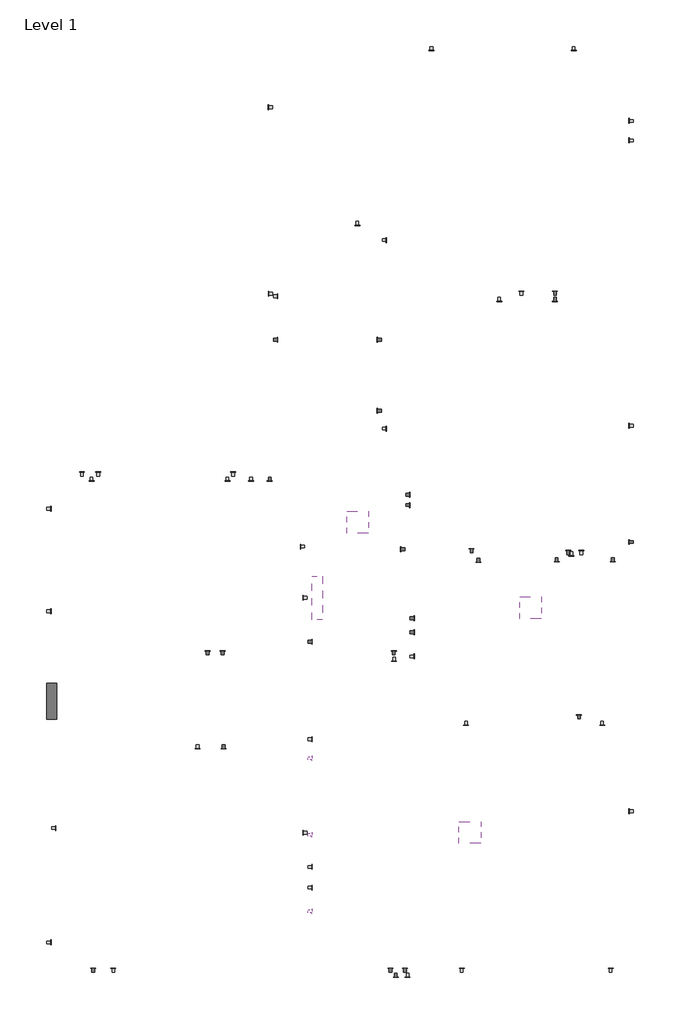
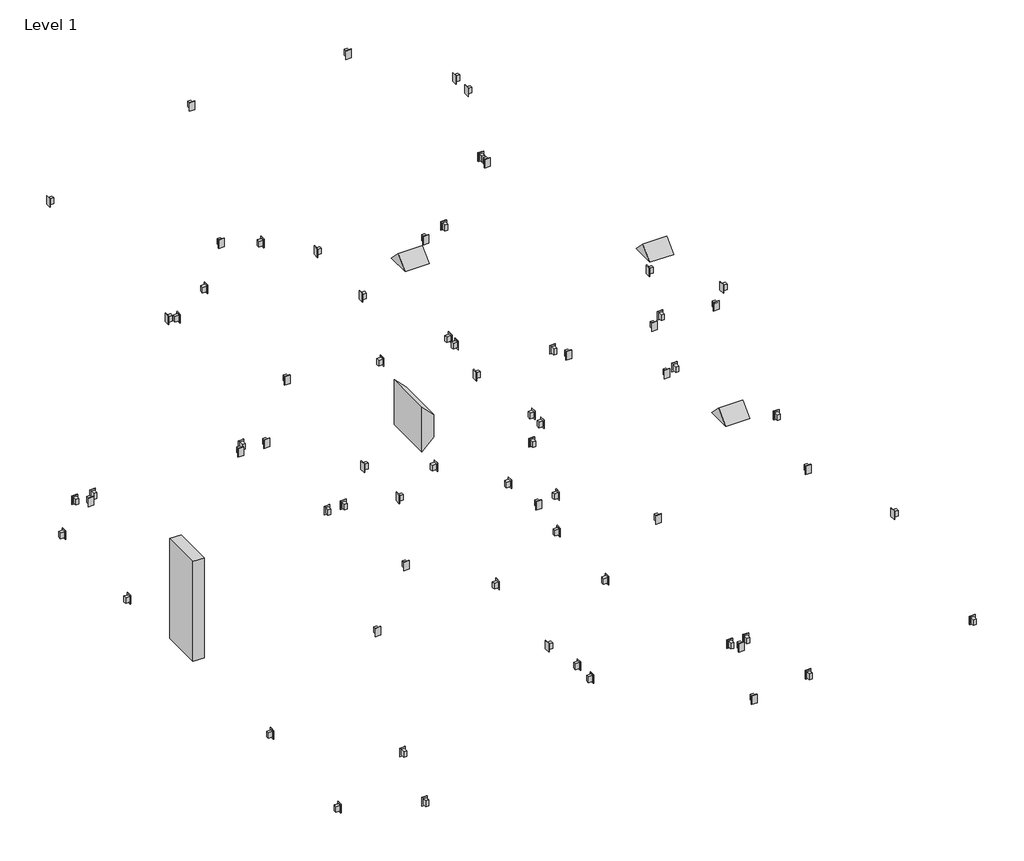
# One storey: 48 proxies, 16 switching devices, 8 electric appliances, 4 light fixtures.
"""IFC4 building model written with IfcOpenShell, lengths in millimetres."""

import ifcopenshell
import ifcopenshell.guid

model = None  # the IFC model being written
_history = None  # IfcOwnerHistory: only IFC2X3 demands one
_inside = {}  # id of a spatial element -> (the spatial element, [elements in it])
_under = {}  # id of a project, library or spatial element -> (it, [spatial elements below it])
_declared = {}  # id of a project -> (the project, [libraries it declares])
_typed = {}  # id of a type object -> (the type object, [elements of that type])
_made_of = {}  # id of a material, layer set ... -> (it, [elements and type objects made of it])


def new_model(schema):
    """Start an empty IFC model of exactly this schema.

    Asked for "IFC4X3", IfcOpenShell would pick the latest addendum, in which some entities
    have other attributes; the version numbers below select the first issue.
    IFC2X3 requires an IfcOwnerHistory on every rooted entity: one is made here for all.
    """
    global model, _history
    if schema == "IFC4X3":
        model = ifcopenshell.file(schema_version=(4, 3, 0, 0))
    else:
        model = ifcopenshell.file(schema=schema)
    _inside.clear()
    _under.clear()
    _declared.clear()
    _typed.clear()
    _made_of.clear()
    _history = None
    if model.schema == "IFC2X3":
        org = make("IfcOrganization", Name="unknown")
        user = make(
            "IfcPersonAndOrganization",
            ThePerson=make("IfcPerson", FamilyName="unknown"),
            TheOrganization=org,
        )
        app = make(
            "IfcApplication",
            ApplicationDeveloper=org,
            Version="unknown",
            ApplicationFullName="unknown",
            ApplicationIdentifier="unknown",
        )
        _history = make(
            "IfcOwnerHistory",
            OwningUser=user,
            OwningApplication=app,
            ChangeAction="ADDED",
            CreationDate=0,
        )
    return model


def make(cls, **values):
    """One entity of the class cls with the attributes given. An attribute that is None is left unset."""
    return model.create_entity(
        cls, **{name: value for name, value in values.items() if value is not None}
    )


def rooted(cls, **values):
    """An entity with a GlobalId (a new one), such as an element, a storey or a relation."""
    return make(cls, GlobalId=ifcopenshell.guid.new(), OwnerHistory=_history, **values)


def si_unit(unit_type, name, prefix=None):
    """IfcSIUnit, for example si_unit("LENGTHUNIT", "METRE", prefix="MILLI")."""
    return make("IfcSIUnit", UnitType=unit_type, Prefix=prefix, Name=name)


def assignment(units):
    """IfcUnitAssignment: the units of a project."""
    return None if units is None else make("IfcUnitAssignment", Units=units)


def point(xyz):
    """IfcCartesianPoint."""
    return None if xyz is None else make("IfcCartesianPoint", Coordinates=xyz)


def direction(xyz):
    """IfcDirection."""
    return None if xyz is None else make("IfcDirection", DirectionRatios=xyz)


def frame(location, z_axis=None, x_axis=None):
    """IfcAxis2Placement3D, a coordinate frame: its origin and axes. An axis left out is left unset."""
    return make(
        "IfcAxis2Placement3D",
        Location=point(location),
        Axis=direction(z_axis),
        RefDirection=direction(x_axis),
    )


def origin():
    """The frame at (0, 0, 0) with its axes left unset."""
    return frame((0.0, 0.0, 0.0))


def origin_with_axes():
    """The frame at (0, 0, 0) with the z axis (0, 0, 1) and the x axis (1, 0, 0) written out."""
    return frame((0.0, 0.0, 0.0), z_axis=(0.0, 0.0, 1.0), x_axis=(1.0, 0.0, 0.0))


def place(relative_to, where):
    """IfcLocalPlacement: puts the frame where relative to a parent placement (None: the world)."""
    return make(
        "IfcLocalPlacement", PlacementRelTo=relative_to, RelativePlacement=where
    )


def context(
    kind, dimensions, precision=None, world=None, true_north=None, identifier=None
):
    """IfcGeometricRepresentationContext, for example the 3D "Model" context."""
    return make(
        "IfcGeometricRepresentationContext",
        ContextIdentifier=identifier,
        ContextType=kind,
        CoordinateSpaceDimension=dimensions,
        Precision=precision,
        WorldCoordinateSystem=world,
        TrueNorth=true_north,
    )


def project(units=None, contexts=None):
    """IfcProject with its units and contexts."""
    return rooted(
        "IfcProject",
        Name="project",
        RepresentationContexts=contexts,
        UnitsInContext=assignment(units),
    )


def spatial(cls, under=None, at=None, **own):
    """A site, building, storey or space (cls), placed at a placement, below another one or the project."""
    s = rooted(cls, ObjectPlacement=at, **own)
    if under is not None:
        _under.setdefault(under.id(), (under, []))[1].append(s)
    return s


def polyline(points):
    """IfcPolyline through the points."""
    return make("IfcPolyline", Points=[point(p) for p in points])


def outline(outer, holes=None, kind="AREA"):
    """IfcArbitraryClosedProfileDef: a profile drawn as a closed curve; with holes, ...WithVoids."""
    if holes is None:
        return make("IfcArbitraryClosedProfileDef", ProfileType=kind, OuterCurve=outer)
    return make(
        "IfcArbitraryProfileDefWithVoids",
        ProfileType=kind,
        OuterCurve=outer,
        InnerCurves=holes,
    )


def extrude(swept, where, along, depth):
    """IfcExtrudedAreaSolid: the profile swept, set in the frame where, extruded along a direction by depth."""
    return make(
        "IfcExtrudedAreaSolid",
        SweptArea=swept,
        Position=where,
        ExtrudedDirection=direction(along),
        Depth=depth,
    )


def shape(context_of_items, identifier, shape_type, items):
    """IfcShapeRepresentation: the items that make up one representation, for example the "Body"."""
    return make(
        "IfcShapeRepresentation",
        ContextOfItems=context_of_items,
        RepresentationIdentifier=identifier,
        RepresentationType=shape_type,
        Items=items,
    )


def source(mapping_origin, context_of_items, identifier, shape_type, items):
    """IfcRepresentationMap: a shape defined once, which mapped items show again and again."""
    return make(
        "IfcRepresentationMap",
        MappingOrigin=mapping_origin,
        MappedRepresentation=shape(context_of_items, identifier, shape_type, items),
    )


def transform(
    local_origin,
    x_axis=None,
    y_axis=None,
    z_axis=None,
    scale=None,
    scale2=None,
    scale3=None,
    uniform=True,
):
    """IfcCartesianTransformationOperator3D, or its non-uniform kind. x_axis, y_axis, z_axis: its Axis1, 2, 3."""
    if uniform:
        return make(
            "IfcCartesianTransformationOperator3D",
            Axis1=direction(x_axis),
            Axis2=direction(y_axis),
            LocalOrigin=point(local_origin),
            Scale=scale,
            Axis3=direction(z_axis),
        )
    return make(
        "IfcCartesianTransformationOperator3DnonUniform",
        Axis1=direction(x_axis),
        Axis2=direction(y_axis),
        LocalOrigin=point(local_origin),
        Scale=scale,
        Axis3=direction(z_axis),
        Scale2=scale2,
        Scale3=scale3,
    )


def mapped(mapping_source, mapping_target):
    """IfcMappedItem: shows the shape of a source again, moved by a transform."""
    return make(
        "IfcMappedItem", MappingSource=mapping_source, MappingTarget=mapping_target
    )


def made_of(thing, what):
    """Note that an element or type object is made of a material, layer set ...; save() writes the relation."""
    if what is not None:
        _made_of.setdefault(what.id(), (what, []))[1].append(thing)
    return thing


def element(
    cls,
    number,
    at=None,
    inside=None,
    cuts=None,
    type_object=None,
    material=None,
    context=None,
    identifier="Body",
    shape_type=None,
    held_by="IfcProductDefinitionShape",
    body=None,
    shapes=None,
    **own,
):
    """One element of the class cls, such as IfcWall. Its Tag is "e" and its number.

    at: its placement. inside: the storey or other place that contains it. cuts: it is an
    opening in that element (IfcRelVoidsElement). A single representation is given by context,
    identifier, shape_type and body (its items); several are given by shapes. held_by: the class
    of the entity that holds the representations. save() writes the other relations.
    """
    e = rooted(cls, Tag="e%d" % number, ObjectPlacement=at, **own)
    if body is not None:
        shapes = [shape(context, identifier, shape_type, body)]
    if shapes is not None:
        e.Representation = make(held_by, Representations=shapes)
    if inside is not None:
        _inside.setdefault(inside.id(), (inside, []))[1].append(e)
    if cuts is not None:
        rooted(
            "IfcRelVoidsElement", RelatingBuildingElement=cuts, RelatedOpeningElement=e
        )
    if type_object is not None:
        _typed.setdefault(type_object.id(), (type_object, []))[1].append(e)
    return made_of(e, material)


def aggregate(whole, parts):
    """IfcRelAggregates: a whole, such as a stair, and the parts it consists of."""
    return rooted("IfcRelAggregates", RelatingObject=whole, RelatedObjects=parts)


def save(model, path):
    """Write the relations noted so far, then the file.

    IfcRelAggregates (storeys below a building ...), IfcRelContainedInSpatialStructure (elements
    in a storey), IfcRelDefinesByType, IfcRelAssociatesMaterial and IfcRelDeclares: one each for
    every whole, place, type object, material and project.
    """
    for whole, parts in _under.values():
        aggregate(whole, parts)
    for where, things in _inside.values():
        rooted(
            "IfcRelContainedInSpatialStructure",
            RelatedElements=things,
            RelatingStructure=where,
        )
    for kind, things in _typed.values():
        rooted("IfcRelDefinesByType", RelatedObjects=things, RelatingType=kind)
    for what, things in _made_of.values():
        rooted("IfcRelAssociatesMaterial", RelatedObjects=things, RelatingMaterial=what)
    for by, libraries in _declared.values():
        rooted("IfcRelDeclares", RelatingContext=by, RelatedDefinitions=libraries)
    model.write(path)


def duplex_receptacle_gfci_10251bba(model_context):
    return source(origin(), model_context, "Body", "SweptSolid", [
        extrude(outline(polyline([(19.05, 38.1), (19.05, -38.1), (-19.05, -38.1), (-19.05, 38.1), (19.05, 38.1)])), frame((0.0, 0.0, -53.975), z_axis=(0.0, 0.0, 1.0), x_axis=(1.0, 0.0, 0.0)), (0.0, 0.0, 1.0), 53.975),
        extrude(outline(polyline([(34.925, 57.15), (34.925, -57.15), (-34.925, -57.15), (-34.925, 57.15), (34.925, 57.15)])), origin_with_axes(), (0.0, 0.0, 1.0), 4.7625),
    ])


def lighting_and_appliance_panelboard_208v_mlo_400_a_bd3ac378(model_context):
    return source(origin(), model_context, "Body", "SweptSolid", [
        extrude(outline(polyline([(254.0, 673.1), (254.0, -673.1), (-254.0, -673.1), (-254.0, 673.1), (254.0, 673.1)])), frame((0.0, 0.0, -146.05), z_axis=(0.0, 0.0, 1.0), x_axis=(1.0, 0.0, 0.0)), (0.0, 0.0, 1.0), 146.05),
    ])


def data_outlet_plain_367a9a66(model_context):
    return source(origin(), model_context, "Body", "SweptSolid", [
        extrude(outline(polyline([(34.925, 57.15), (34.925, -57.15), (-34.925, -57.15), (-34.925, 57.15), (34.925, 57.15)])), origin_with_axes(), (0.0, 0.0, 1.0), 4.7625),
        extrude(outline(polyline([(19.05, 38.1), (19.05, -38.1), (-19.05, -38.1), (-19.05, 38.1), (19.05, 38.1)])), frame((0.0, 0.0, -53.975), z_axis=(0.0, 0.0, 1.0), x_axis=(1.0, 0.0, 0.0)), (0.0, 0.0, 1.0), 53.975),
    ])


def plain_recessed_lighting_fixture_2x2_120_2107ce2d(model_context):
    return source(origin(), model_context, "Body", "SweptSolid", [
        extrude(outline(polyline([(-609.6, 0.0), (0.0, 0.0), (-152.4, -152.4), (-457.2, -152.4), (-609.6, 0.0)])), frame((0.0, 0.0, 0.0), z_axis=(1.0, 0.0, 0.0), x_axis=(0.0, 1.0, 0.0)), (0.0, 0.0, 1.0), 609.6),
    ])


def plain_recessed_lighting_fixture_large_bulb_b9741ada(model_context):
    return source(origin(), model_context, "Body", "SweptSolid", [
        extrude(outline(polyline([(-304.8, 0.0), (0.0, 0.0), (-152.4, -152.4), (-304.8, 0.0)])), frame((0.0, 0.0, 0.0), z_axis=(1.0, 0.0, 0.0), x_axis=(0.0, 1.0, 0.0)), (0.0, 0.0, 1.0), 304.8),
    ])


model = new_model("IFC4")

# Units and contexts
model_context = context("Model", 3, world=origin())
ifc_project = project(units=[si_unit("LENGTHUNIT", "METRE", prefix="MILLI")], contexts=[model_context])

# Site, building, storey
site = spatial("IfcSite", under=ifc_project)
building = spatial("IfcBuilding", under=site)
storey = spatial("IfcBuildingStorey", under=building, Name="Level 1", Elevation=0.0)

# Proxies
placement = place(None, origin())
duplex_receptacle_gfci_shape = duplex_receptacle_gfci_10251bba(model_context)
element("IfcBuildingElementProxy", 1, Name="Duplex Receptacle : GFCI", ObjectType="Duplex Receptacle : GFCI", at=placement, inside=storey, context=model_context, shape_type="MappedRepresentation", body=[
    mapped(duplex_receptacle_gfci_shape, transform((-384.264748, 4509.2322925, 1219.2), x_axis=(0.0, 1.0, 0.0), y_axis=(0.0, 0.0, 1.0), z_axis=(1.0, 0.0, 0.0))),
])
element("IfcBuildingElementProxy", 2, Name="Duplex Receptacle : GFCI", ObjectType="Duplex Receptacle : GFCI", at=placement, inside=storey, context=model_context, shape_type="MappedRepresentation", body=[
    mapped(duplex_receptacle_gfci_shape, transform((-384.264748, 4707.743975, 1219.2), x_axis=(0.0, 1.0, 0.0), y_axis=(0.0, 0.0, 1.0), z_axis=(1.0, 0.0, 0.0))),
])
element("IfcBuildingElementProxy", 3, Name="Duplex Receptacle : GFCI", ObjectType="Duplex Receptacle : GFCI", at=placement, inside=storey, context=model_context, shape_type="MappedRepresentation", body=[
    mapped(duplex_receptacle_gfci_shape, transform((520.3675151, 5493.8871474, 1219.2), x_axis=(1.0, 0.0, 0.0), y_axis=(0.0, 0.0, 1.0), z_axis=(0.0, -1.0, 0.0))),
])
element("IfcBuildingElementProxy", 4, Name="Duplex Receptacle : GFCI", ObjectType="Duplex Receptacle : GFCI", at=placement, inside=storey, context=model_context, shape_type="MappedRepresentation", body=[
    mapped(duplex_receptacle_gfci_shape, transform((1616.819892, 5500.2371474, 1219.2), x_axis=(1.0, 0.0, 0.0), y_axis=(0.0, 0.0, 1.0), z_axis=(0.0, -1.0, 0.0))),
])
element("IfcBuildingElementProxy", 5, Name="Duplex Receptacle : GFCI", ObjectType="Duplex Receptacle : GFCI", at=placement, inside=storey, context=model_context, shape_type="MappedRepresentation", body=[
    mapped(duplex_receptacle_gfci_shape, transform((2401.5903749, 5500.2371474, 1219.2), x_axis=(1.0, 0.0, 0.0), y_axis=(0.0, 0.0, 1.0), z_axis=(0.0, -1.0, 0.0))),
])
element("IfcBuildingElementProxy", 6, Name="Duplex Receptacle : GFCI", ObjectType="Duplex Receptacle : GFCI", at=placement, inside=storey, context=model_context, shape_type="MappedRepresentation", body=[
    mapped(duplex_receptacle_gfci_shape, transform((-444.589748, 6434.9811372, 1219.2), x_axis=(0.0, 1.0, 0.0), y_axis=(0.0, 0.0, 1.0), z_axis=(1.0, 0.0, 0.0))),
])
element("IfcBuildingElementProxy", 7, Name="Duplex Receptacle : GFCI", ObjectType="Duplex Receptacle : GFCI", at=placement, inside=storey, context=model_context, shape_type="MappedRepresentation", body=[
    mapped(duplex_receptacle_gfci_shape, transform((-444.589748, 6292.1269358, 1219.2), x_axis=(0.0, 1.0, 0.0), y_axis=(0.0, 0.0, 1.0), z_axis=(1.0, 0.0, 0.0))),
])
element("IfcBuildingElementProxy", 8, Name="Duplex Receptacle : GFCI", ObjectType="Duplex Receptacle : GFCI", at=placement, inside=storey, context=model_context, shape_type="MappedRepresentation", body=[
    mapped(duplex_receptacle_gfci_shape, transform((423.8945479, 5678.0371474, 1219.2), x_axis=(-1.0, 0.0, 0.0), y_axis=(0.0, 0.0, 1.0), z_axis=(0.0, 1.0, 0.0))),
])
element("IfcBuildingElementProxy", 9, Name="Duplex Receptacle : GFCI", ObjectType="Duplex Receptacle : GFCI", at=placement, inside=storey, context=model_context, shape_type="MappedRepresentation", body=[
    mapped(duplex_receptacle_gfci_shape, transform((1778.2265871, 5652.6371474, 1219.2), x_axis=(-1.0, 0.0, 0.0), y_axis=(0.0, 0.0, 1.0), z_axis=(0.0, 1.0, 0.0))),
])
element("IfcBuildingElementProxy", 10, Name="Duplex Receptacle : GFCI", ObjectType="Duplex Receptacle : GFCI", at=placement, inside=storey, context=model_context, shape_type="MappedRepresentation", body=[
    mapped(duplex_receptacle_gfci_shape, transform((2635.160252, 5774.512362, 1219.2), x_axis=(0.0, -1.0, 0.0), y_axis=(0.0, 0.0, 1.0), z_axis=(-1.0, 0.0, 0.0))),
])
element("IfcBuildingElementProxy", 11, Name="Duplex Receptacle : GFCI", ObjectType="Duplex Receptacle : GFCI", at=placement, inside=storey, context=model_context, shape_type="MappedRepresentation", body=[
    mapped(duplex_receptacle_gfci_shape, transform((-1816.189748, 4378.2462129, 1219.2), x_axis=(0.0, 1.0, 0.0), y_axis=(0.0, 0.0, 1.0), z_axis=(1.0, 0.0, 0.0))),
])
element("IfcBuildingElementProxy", 12, Name="Duplex Receptacle : Standard", ObjectType="Duplex Receptacle : Standard", at=placement, inside=storey, context=model_context, shape_type="MappedRepresentation", body=[
    mapped(duplex_receptacle_gfci_shape, transform((-5473.789748, 4805.3855798, 457.2), x_axis=(0.0, 1.0, 0.0), y_axis=(0.0, 0.0, 1.0), z_axis=(1.0, 0.0, 0.0))),
])
element("IfcBuildingElementProxy", 13, Name="Duplex Receptacle : Standard", ObjectType="Duplex Receptacle : Standard", at=placement, inside=storey, context=model_context, shape_type="MappedRepresentation", body=[
    mapped(duplex_receptacle_gfci_shape, transform((-5473.789748, 6239.7970199, 457.2), x_axis=(0.0, 1.0, 0.0), y_axis=(0.0, 0.0, 1.0), z_axis=(1.0, 0.0, 0.0))),
])
element("IfcBuildingElementProxy", 14, Name="Duplex Receptacle : Standard", ObjectType="Duplex Receptacle : Standard", at=placement, inside=storey, context=model_context, shape_type="MappedRepresentation", body=[
    mapped(duplex_receptacle_gfci_shape, transform((-4904.2560493, 6630.4078904, 457.2), x_axis=(1.0, 0.0, 0.0), y_axis=(0.0, 0.0, 1.0), z_axis=(0.0, -1.0, 0.0))),
])
element("IfcBuildingElementProxy", 15, Name="Duplex Receptacle : Standard", ObjectType="Duplex Receptacle : Standard", at=placement, inside=storey, context=model_context, shape_type="MappedRepresentation", body=[
    mapped(duplex_receptacle_gfci_shape, transform((-2998.0299372, 6630.4078904, 457.2), x_axis=(1.0, 0.0, 0.0), y_axis=(0.0, 0.0, 1.0), z_axis=(0.0, -1.0, 0.0))),
])
element("IfcBuildingElementProxy", 16, Name="Duplex Receptacle : Standard", ObjectType="Duplex Receptacle : Standard", at=placement, inside=storey, context=model_context, shape_type="MappedRepresentation", body=[
    mapped(duplex_receptacle_gfci_shape, transform((-2666.1000171, 6630.4078904, 457.2), x_axis=(1.0, 0.0, 0.0), y_axis=(0.0, 0.0, 1.0), z_axis=(0.0, -1.0, 0.0))),
])
element("IfcBuildingElementProxy", 17, Name="Duplex Receptacle : Standard", ObjectType="Duplex Receptacle : Standard", at=placement, inside=storey, context=model_context, shape_type="MappedRepresentation", body=[
    mapped(duplex_receptacle_gfci_shape, transform((-1936.839748, 4995.0598198, 457.2), x_axis=(0.0, -1.0, 0.0), y_axis=(0.0, 0.0, 1.0), z_axis=(-1.0, 0.0, 0.0))),
])
element("IfcBuildingElementProxy", 18, Name="Duplex Receptacle : Standard", ObjectType="Duplex Receptacle : Standard", at=placement, inside=storey, context=model_context, shape_type="MappedRepresentation", body=[
    mapped(duplex_receptacle_gfci_shape, transform((-3414.9283858, 2880.8621474, 457.2), x_axis=(1.0, 0.0, 0.0), y_axis=(0.0, 0.0, 1.0), z_axis=(0.0, -1.0, 0.0))),
])
element("IfcBuildingElementProxy", 19, Name="Duplex Receptacle : Standard", ObjectType="Duplex Receptacle : Standard", at=placement, inside=storey, context=model_context, shape_type="MappedRepresentation", body=[
    mapped(duplex_receptacle_gfci_shape, transform((-1936.839748, 1703.0761834, 457.2), x_axis=(0.0, -1.0, 0.0), y_axis=(0.0, 0.0, 1.0), z_axis=(-1.0, 0.0, 0.0))),
])
element("IfcBuildingElementProxy", 20, Name="Duplex Receptacle : Standard", ObjectType="Duplex Receptacle : Standard", at=placement, inside=storey, context=model_context, shape_type="MappedRepresentation", body=[
    mapped(duplex_receptacle_gfci_shape, transform((-4597.0361882, -198.8878526, 457.2), x_axis=(-1.0, 0.0, 0.0), y_axis=(0.0, 0.0, 1.0), z_axis=(0.0, 1.0, 0.0))),
])
element("IfcBuildingElementProxy", 21, Name="Duplex Receptacle : Standard", ObjectType="Duplex Receptacle : Standard", at=placement, inside=storey, context=model_context, shape_type="MappedRepresentation", body=[
    mapped(duplex_receptacle_gfci_shape, transform((-5407.114748, 1768.3250081, 457.2), x_axis=(0.0, 1.0, 0.0), y_axis=(0.0, 0.0, 1.0), z_axis=(1.0, 0.0, 0.0))),
])
element("IfcBuildingElementProxy", 22, Name="Duplex Receptacle : Standard", ObjectType="Duplex Receptacle : Standard", at=placement, inside=storey, context=model_context, shape_type="MappedRepresentation", body=[
    mapped(duplex_receptacle_gfci_shape, transform((-1816.189748, 2744.9323475, 1981.2), x_axis=(0.0, 1.0, 0.0), y_axis=(0.0, 0.0, 1.0), z_axis=(1.0, 0.0, 0.0))),
])
element("IfcBuildingElementProxy", 23, Name="Duplex Receptacle : Standard", ObjectType="Duplex Receptacle : Standard", at=placement, inside=storey, context=model_context, shape_type="MappedRepresentation", body=[
    mapped(duplex_receptacle_gfci_shape, transform((-1816.189748, 1673.8457407, 1981.2), x_axis=(0.0, 1.0, 0.0), y_axis=(0.0, 0.0, 1.0), z_axis=(1.0, 0.0, 0.0))),
])
element("IfcBuildingElementProxy", 24, Name="Duplex Receptacle : Standard", ObjectType="Duplex Receptacle : Standard", at=placement, inside=storey, context=model_context, shape_type="MappedRepresentation", body=[
    mapped(duplex_receptacle_gfci_shape, transform((-1816.189748, 602.759134, 1981.2), x_axis=(0.0, 1.0, 0.0), y_axis=(0.0, 0.0, 1.0), z_axis=(1.0, 0.0, 0.0))),
])
element("IfcBuildingElementProxy", 25, Name="Duplex Receptacle : Standard", ObjectType="Duplex Receptacle : Standard", at=placement, inside=storey, context=model_context, shape_type="MappedRepresentation", body=[
    mapped(duplex_receptacle_gfci_shape, transform((-1816.189748, 1223.3093109, 457.2), x_axis=(0.0, 1.0, 0.0), y_axis=(0.0, 0.0, 1.0), z_axis=(1.0, 0.0, 0.0))),
])
element("IfcBuildingElementProxy", 26, Name="Duplex Receptacle : Standard", ObjectType="Duplex Receptacle : Standard", at=placement, inside=storey, context=model_context, shape_type="MappedRepresentation", body=[
    mapped(duplex_receptacle_gfci_shape, transform((-384.264748, 4171.5769074, 457.2), x_axis=(0.0, 1.0, 0.0), y_axis=(0.0, 0.0, 1.0), z_axis=(1.0, 0.0, 0.0))),
])
element("IfcBuildingElementProxy", 27, Name="Duplex Receptacle : Standard", ObjectType="Duplex Receptacle : Standard", at=placement, inside=storey, context=model_context, shape_type="MappedRepresentation", body=[
    mapped(duplex_receptacle_gfci_shape, transform((-473.2412845, -319.5378526, 457.2), x_axis=(1.0, 0.0, 0.0), y_axis=(0.0, 0.0, 1.0), z_axis=(0.0, -1.0, 0.0))),
])
element("IfcBuildingElementProxy", 28, Name="Duplex Receptacle : Standard", ObjectType="Duplex Receptacle : Standard", at=placement, inside=storey, context=model_context, shape_type="MappedRepresentation", body=[
    mapped(duplex_receptacle_gfci_shape, transform((-661.5219929, 4106.2828904, 457.2), x_axis=(1.0, 0.0, 0.0), y_axis=(0.0, 0.0, 1.0), z_axis=(0.0, -1.0, 0.0))),
])
element("IfcBuildingElementProxy", 29, Name="Duplex Receptacle : Standard", ObjectType="Duplex Receptacle : Standard", at=placement, inside=storey, context=model_context, shape_type="MappedRepresentation", body=[
    mapped(duplex_receptacle_gfci_shape, transform((345.9891561, 3210.9328904, 457.2), x_axis=(1.0, 0.0, 0.0), y_axis=(0.0, 0.0, 1.0), z_axis=(0.0, -1.0, 0.0))),
])
element("IfcBuildingElementProxy", 30, Name="Duplex Receptacle : Standard", ObjectType="Duplex Receptacle : Standard", at=placement, inside=storey, context=model_context, shape_type="MappedRepresentation", body=[
    mapped(duplex_receptacle_gfci_shape, transform((2252.7417537, 3210.9328904, 457.2), x_axis=(1.0, 0.0, 0.0), y_axis=(0.0, 0.0, 1.0), z_axis=(0.0, -1.0, 0.0))),
])
element("IfcBuildingElementProxy", 31, Name="Duplex Receptacle : Standard", ObjectType="Duplex Receptacle : Standard", at=placement, inside=storey, context=model_context, shape_type="MappedRepresentation", body=[
    mapped(duplex_receptacle_gfci_shape, transform((2635.160252, 2005.0564649, 457.2), x_axis=(0.0, -1.0, 0.0), y_axis=(0.0, 0.0, 1.0), z_axis=(-1.0, 0.0, 0.0))),
])
element("IfcBuildingElementProxy", 32, Name="Duplex Receptacle : Standard", ObjectType="Duplex Receptacle : Standard", at=placement, inside=storey, context=model_context, shape_type="MappedRepresentation", body=[
    mapped(duplex_receptacle_gfci_shape, transform((2372.6222976, -198.8878526, 457.2), x_axis=(-1.0, 0.0, 0.0), y_axis=(0.0, 0.0, 1.0), z_axis=(0.0, 1.0, 0.0))),
])
element("IfcBuildingElementProxy", 33, Name="Duplex Receptacle : Standard", ObjectType="Duplex Receptacle : Standard", at=placement, inside=storey, context=model_context, shape_type="MappedRepresentation", body=[
    mapped(duplex_receptacle_gfci_shape, transform((284.9208673, -198.8878526, 457.2), x_axis=(-1.0, 0.0, 0.0), y_axis=(0.0, 0.0, 1.0), z_axis=(0.0, 1.0, 0.0))),
])
element("IfcBuildingElementProxy", 34, Name="Duplex Receptacle : Standard", ObjectType="Duplex Receptacle : Standard", at=placement, inside=storey, context=model_context, shape_type="MappedRepresentation", body=[
    mapped(duplex_receptacle_gfci_shape, transform((-138.4982364, 12659.8621474, 457.2), x_axis=(1.0, 0.0, 0.0), y_axis=(0.0, 0.0, 1.0), z_axis=(0.0, -1.0, 0.0))),
])
element("IfcBuildingElementProxy", 35, Name="Duplex Receptacle : Standard", ObjectType="Duplex Receptacle : Standard", at=placement, inside=storey, context=model_context, shape_type="MappedRepresentation", body=[
    mapped(duplex_receptacle_gfci_shape, transform((1854.1028631, 12659.8621474, 457.2), x_axis=(1.0, 0.0, 0.0), y_axis=(0.0, 0.0, 1.0), z_axis=(0.0, -1.0, 0.0))),
])
element("IfcBuildingElementProxy", 36, Name="Duplex Receptacle : Standard", ObjectType="Duplex Receptacle : Standard", at=placement, inside=storey, context=model_context, shape_type="MappedRepresentation", body=[
    mapped(duplex_receptacle_gfci_shape, transform((2635.160252, 11398.5773679, 457.2), x_axis=(0.0, -1.0, 0.0), y_axis=(0.0, 0.0, 1.0), z_axis=(-1.0, 0.0, 0.0))),
])
element("IfcBuildingElementProxy", 37, Name="Duplex Receptacle : Standard", ObjectType="Duplex Receptacle : Standard", at=placement, inside=storey, context=model_context, shape_type="MappedRepresentation", body=[
    mapped(duplex_receptacle_gfci_shape, transform((1121.4544653, 9284.8371474, 457.2), x_axis=(-1.0, 0.0, 0.0), y_axis=(0.0, 0.0, 1.0), z_axis=(0.0, 1.0, 0.0))),
])
element("IfcBuildingElementProxy", 38, Name="Duplex Receptacle : Standard", ObjectType="Duplex Receptacle : Standard", at=placement, inside=storey, context=model_context, shape_type="MappedRepresentation", body=[
    mapped(duplex_receptacle_gfci_shape, transform((-774.789748, 10004.0725015, 457.2), x_axis=(0.0, 1.0, 0.0), y_axis=(0.0, 0.0, 1.0), z_axis=(1.0, 0.0, 0.0))),
])
element("IfcBuildingElementProxy", 39, Name="Duplex Receptacle : Standard", ObjectType="Duplex Receptacle : Standard", at=placement, inside=storey, context=model_context, shape_type="MappedRepresentation", body=[
    mapped(duplex_receptacle_gfci_shape, transform((810.2121097, 9145.1371474, 457.2), x_axis=(1.0, 0.0, 0.0), y_axis=(0.0, 0.0, 1.0), z_axis=(0.0, -1.0, 0.0))),
])
element("IfcBuildingElementProxy", 40, Name="Duplex Receptacle : Standard", ObjectType="Duplex Receptacle : Standard", at=placement, inside=storey, context=model_context, shape_type="MappedRepresentation", body=[
    mapped(duplex_receptacle_gfci_shape, transform((2635.160252, 7402.2491499, 457.2), x_axis=(0.0, -1.0, 0.0), y_axis=(0.0, 0.0, 1.0), z_axis=(-1.0, 0.0, 0.0))),
])
element("IfcBuildingElementProxy", 41, Name="Duplex Receptacle : Standard", ObjectType="Duplex Receptacle : Standard", at=placement, inside=storey, context=model_context, shape_type="MappedRepresentation", body=[
    mapped(duplex_receptacle_gfci_shape, transform((-774.789748, 7363.5981384, 457.2), x_axis=(0.0, 1.0, 0.0), y_axis=(0.0, 0.0, 1.0), z_axis=(1.0, 0.0, 0.0))),
])
element("IfcBuildingElementProxy", 42, Name="Duplex Receptacle : Standard", ObjectType="Duplex Receptacle : Standard", at=placement, inside=storey, context=model_context, shape_type="MappedRepresentation", body=[
    mapped(duplex_receptacle_gfci_shape, transform((-2298.789748, 9216.6288333, 457.2), x_axis=(0.0, 1.0, 0.0), y_axis=(0.0, 0.0, 1.0), z_axis=(1.0, 0.0, 0.0))),
])
element("IfcBuildingElementProxy", 43, Name="Duplex Receptacle : Standard", ObjectType="Duplex Receptacle : Standard", at=placement, inside=storey, context=model_context, shape_type="MappedRepresentation", body=[
    mapped(duplex_receptacle_gfci_shape, transform((-5037.5731778, 6751.0578904, 457.2), x_axis=(-1.0, 0.0, 0.0), y_axis=(0.0, 0.0, 1.0), z_axis=(0.0, 1.0, 0.0))),
])
element("IfcBuildingElementProxy", 44, Name="Duplex Receptacle : Standard", ObjectType="Duplex Receptacle : Standard", at=placement, inside=storey, context=model_context, shape_type="MappedRepresentation", body=[
    mapped(duplex_receptacle_gfci_shape, transform((-2920.5988576, 6751.0578904, 457.2), x_axis=(-1.0, 0.0, 0.0), y_axis=(0.0, 0.0, 1.0), z_axis=(0.0, 1.0, 0.0))),
])
element("IfcBuildingElementProxy", 45, Name="Duplex Receptacle : Standard", ObjectType="Duplex Receptacle : Standard", at=placement, inside=storey, context=model_context, shape_type="MappedRepresentation", body=[
    mapped(duplex_receptacle_gfci_shape, transform((-2419.439748, 9250.6845574, 457.2), x_axis=(0.0, -1.0, 0.0), y_axis=(0.0, 0.0, 1.0), z_axis=(-1.0, 0.0, 0.0))),
])
element("IfcBuildingElementProxy", 46, Name="Duplex Receptacle : Standard", ObjectType="Duplex Receptacle : Standard", at=placement, inside=storey, context=model_context, shape_type="MappedRepresentation", body=[
    mapped(duplex_receptacle_gfci_shape, transform((-2422.614748, 11862.2125422, 457.2), x_axis=(0.0, -1.0, 0.0), y_axis=(0.0, 0.0, 1.0), z_axis=(-1.0, 0.0, 0.0))),
])
element("IfcBuildingElementProxy", 47, Name="Duplex Receptacle : Standard", ObjectType="Duplex Receptacle : Standard", at=placement, inside=storey, context=model_context, shape_type="MappedRepresentation", body=[
    mapped(duplex_receptacle_gfci_shape, transform((-1177.5604885, 10211.9371474, 457.2), x_axis=(1.0, 0.0, 0.0), y_axis=(0.0, 0.0, 1.0), z_axis=(0.0, -1.0, 0.0))),
])
lighting_and_appliance_panelboard_208v_mlo_400_a_shape = lighting_and_appliance_panelboard_208v_mlo_400_a_bd3ac378(model_context)
element("IfcBuildingElementProxy", 48, Name="Lighting and Appliance Panelboard - 208V MLO : 400 A", ObjectType="Lighting and Appliance Panelboard - 208V MLO : 400 A", at=placement, inside=storey, context=model_context, shape_type="MappedRepresentation", body=[
    mapped(lighting_and_appliance_panelboard_208v_mlo_400_a_shape, transform((-5534.114748, 3545.0819838, 1219.2), x_axis=(0.0, -1.0, 0.0), y_axis=(0.0, 0.0, 1.0), z_axis=(-1.0, 0.0, 0.0))),
])

# Electric appliances
data_outlet_plain_shape = data_outlet_plain_367a9a66(model_context)
element("IfcElectricAppliance", 49, ObjectType="Data Outlet : Plain", at=placement, inside=storey, context=model_context, shape_type="MappedRepresentation", body=[
    mapped(data_outlet_plain_shape, transform((-1816.189748, 934.2859408, 457.2), x_axis=(0.0, 1.0, 0.0), y_axis=(0.0, 0.0, 1.0), z_axis=(1.0, 0.0, 0.0))),
])
element("IfcElectricAppliance", 50, ObjectType="Data Outlet : Plain", at=placement, inside=storey, context=model_context, shape_type="MappedRepresentation", body=[
    mapped(data_outlet_plain_shape, transform((-1816.189748, 3012.7039992, 457.2), x_axis=(0.0, 1.0, 0.0), y_axis=(0.0, 0.0, 1.0), z_axis=(1.0, 0.0, 0.0))),
])
element("IfcElectricAppliance", 51, ObjectType="Data Outlet : Plain", at=placement, inside=storey, context=model_context, shape_type="MappedRepresentation", body=[
    mapped(data_outlet_plain_shape, transform((-1971.764748, 5710.8654743, 457.2), x_axis=(0.0, -1.0, 0.0), y_axis=(0.0, 0.0, 1.0), z_axis=(-1.0, 0.0, 0.0))),
])
element("IfcElectricAppliance", 52, ObjectType="Data Outlet : Plain", at=placement, inside=storey, context=model_context, shape_type="MappedRepresentation", body=[
    mapped(data_outlet_plain_shape, transform((-5473.789748, 167.0263887, 457.2), x_axis=(0.0, 1.0, 0.0), y_axis=(0.0, 0.0, 1.0), z_axis=(1.0, 0.0, 0.0))),
])
element("IfcElectricAppliance", 53, ObjectType="Data Outlet : Plain", at=placement, inside=storey, context=model_context, shape_type="MappedRepresentation", body=[
    mapped(data_outlet_plain_shape, transform((1824.2195174, 5582.7871474, 457.2), x_axis=(1.0, 0.0, 0.0), y_axis=(0.0, 0.0, 1.0), z_axis=(0.0, -1.0, 0.0))),
])
element("IfcElectricAppliance", 54, ObjectType="Data Outlet : Plain", at=placement, inside=storey, context=model_context, shape_type="MappedRepresentation", body=[
    mapped(data_outlet_plain_shape, transform((1963.2054307, 5652.6371474, 457.2), x_axis=(-1.0, 0.0, 0.0), y_axis=(0.0, 0.0, 1.0), z_axis=(0.0, 1.0, 0.0))),
])
element("IfcElectricAppliance", 55, ObjectType="Data Outlet : Plain", at=placement, inside=storey, context=model_context, shape_type="MappedRepresentation", body=[
    mapped(data_outlet_plain_shape, transform((2635.160252, 11671.585365, 457.2), x_axis=(0.0, -1.0, 0.0), y_axis=(0.0, 0.0, 1.0), z_axis=(-1.0, 0.0, 0.0))),
])
element("IfcElectricAppliance", 56, ObjectType="Data Outlet : Plain", at=placement, inside=storey, context=model_context, shape_type="MappedRepresentation", body=[
    mapped(data_outlet_plain_shape, transform((-4810.7942528, 6751.0578904, 457.2), x_axis=(-1.0, 0.0, 0.0), y_axis=(0.0, 0.0, 1.0), z_axis=(0.0, 1.0, 0.0))),
])

# Light fixtures
plain_recessed_lighting_fixture_2x2_120_shape = plain_recessed_lighting_fixture_2x2_120_2107ce2d(model_context)
element("IfcLightFixture", 57, ObjectType="Plain Recessed Lighting Fixture : 2x2 - 120", at=placement, inside=storey, context=model_context, shape_type="MappedRepresentation", body=[
    mapped(plain_recessed_lighting_fixture_2x2_120_shape, transform((-1816.189748, 4682.7679627, 1219.2), x_axis=(0.0, 1.0, 0.0), y_axis=(0.0, 0.0, -1.0), z_axis=(-1.0, 0.0, 0.0))),
])
plain_recessed_lighting_fixture_large_bulb_shape = plain_recessed_lighting_fixture_large_bulb_b9741ada(model_context)
element("IfcLightFixture", 58, ObjectType="Plain Recessed Lighting Fixture : Large Bulb", at=placement, inside=storey, context=model_context, shape_type="MappedRepresentation", body=[
    mapped(plain_recessed_lighting_fixture_large_bulb_shape, transform((1098.2997064, 4702.280537, 2743.2), x_axis=(1.0, 0.0, 0.0), y_axis=(0.0, -1.0, 0.0), z_axis=(0.0, 0.0, -1.0))),
])
element("IfcLightFixture", 59, ObjectType="Plain Recessed Lighting Fixture : Large Bulb", at=placement, inside=storey, context=model_context, shape_type="MappedRepresentation", body=[
    mapped(plain_recessed_lighting_fixture_large_bulb_shape, transform((246.0901194, 1554.3226748, 2743.2), x_axis=(1.0, 0.0, 0.0), y_axis=(0.0, -1.0, 0.0), z_axis=(0.0, 0.0, -1.0))),
])
element("IfcLightFixture", 60, ObjectType="Plain Recessed Lighting Fixture : Large Bulb", at=placement, inside=storey, context=model_context, shape_type="MappedRepresentation", body=[
    mapped(plain_recessed_lighting_fixture_large_bulb_shape, transform((-1325.936978, 5896.5793657, 2743.2), x_axis=(1.0, 0.0, 0.0), y_axis=(0.0, -1.0, 0.0), z_axis=(0.0, 0.0, -1.0))),
])

# Switching devices
element("IfcSwitchingDevice", 61, ObjectType="Lighting Switches : Dimmer", at=placement, inside=storey, context=model_context, shape_type="MappedRepresentation", body=[
    mapped(duplex_receptacle_gfci_shape, transform((-509.1101164, -198.8878526, 1219.2), x_axis=(-1.0, 0.0, 0.0), y_axis=(0.0, 0.0, 1.0), z_axis=(0.0, 1.0, 0.0))),
])
element("IfcSwitchingDevice", 62, ObjectType="Lighting Switches : Dimmer", at=placement, inside=storey, context=model_context, shape_type="MappedRepresentation", body=[
    mapped(duplex_receptacle_gfci_shape, transform((-714.096431, -198.8878526, 1219.2), x_axis=(-1.0, 0.0, 0.0), y_axis=(0.0, 0.0, 1.0), z_axis=(0.0, 1.0, 0.0))),
])
element("IfcSwitchingDevice", 63, ObjectType="Lighting Switches : Dimmer", at=placement, inside=storey, context=model_context, shape_type="MappedRepresentation", body=[
    mapped(duplex_receptacle_gfci_shape, transform((-3053.5434186, 2880.8621474, 1219.2), x_axis=(1.0, 0.0, 0.0), y_axis=(0.0, 0.0, 1.0), z_axis=(0.0, -1.0, 0.0))),
])
element("IfcSwitchingDevice", 64, ObjectType="Lighting Switches : Dimmer", at=placement, inside=storey, context=model_context, shape_type="MappedRepresentation", body=[
    mapped(duplex_receptacle_gfci_shape, transform((-4878.8977442, -198.8878526, 1219.2), x_axis=(-1.0, 0.0, 0.0), y_axis=(0.0, 0.0, 1.0), z_axis=(0.0, 1.0, 0.0))),
])
element("IfcSwitchingDevice", 65, ObjectType="Lighting Switches : Dimmer", at=placement, inside=storey, context=model_context, shape_type="MappedRepresentation", body=[
    mapped(duplex_receptacle_gfci_shape, transform((-3066.5584227, 4245.9828904, 1219.2), x_axis=(-1.0, 0.0, 0.0), y_axis=(0.0, 0.0, 1.0), z_axis=(0.0, 1.0, 0.0))),
])
element("IfcSwitchingDevice", 66, ObjectType="Lighting Switches : Dimmer", at=placement, inside=storey, context=model_context, shape_type="MappedRepresentation", body=[
    mapped(duplex_receptacle_gfci_shape, transform((-3274.7984884, 4245.9828904, 1219.2), x_axis=(-1.0, 0.0, 0.0), y_axis=(0.0, 0.0, 1.0), z_axis=(0.0, 1.0, 0.0))),
])
element("IfcSwitchingDevice", 67, ObjectType="Lighting Switches : Dimmer", at=placement, inside=storey, context=model_context, shape_type="MappedRepresentation", body=[
    mapped(duplex_receptacle_gfci_shape, transform((-2405.6446994, 6630.4078904, 1219.2), x_axis=(1.0, 0.0, 0.0), y_axis=(0.0, 0.0, 1.0), z_axis=(0.0, -1.0, 0.0))),
])
element("IfcSwitchingDevice", 68, ObjectType="Lighting Switches : Dimmer", at=placement, inside=storey, context=model_context, shape_type="MappedRepresentation", body=[
    mapped(duplex_receptacle_gfci_shape, transform((1593.0552494, 9145.1371474, 1219.2), x_axis=(1.0, 0.0, 0.0), y_axis=(0.0, 0.0, 1.0), z_axis=(0.0, -1.0, 0.0))),
])
element("IfcSwitchingDevice", 69, ObjectType="Lighting Switches : Dimmer", at=placement, inside=storey, context=model_context, shape_type="MappedRepresentation", body=[
    mapped(duplex_receptacle_gfci_shape, transform((1593.0552494, 9284.8371474, 1219.2), x_axis=(-1.0, 0.0, 0.0), y_axis=(0.0, 0.0, 1.0), z_axis=(0.0, 1.0, 0.0))),
])
element("IfcSwitchingDevice", 70, ObjectType="Lighting Switches : Single Pole", at=placement, inside=storey, context=model_context, shape_type="MappedRepresentation", body=[
    mapped(duplex_receptacle_gfci_shape, transform((1929.3102368, 3350.6328904, 1219.2), x_axis=(-1.0, 0.0, 0.0), y_axis=(0.0, 0.0, 1.0), z_axis=(0.0, 1.0, 0.0))),
])
element("IfcSwitchingDevice", 71, ObjectType="Lighting Switches : Single Pole", at=placement, inside=storey, context=model_context, shape_type="MappedRepresentation", body=[
    mapped(duplex_receptacle_gfci_shape, transform((-639.2601574, -319.5378526, 1219.2), x_axis=(1.0, 0.0, 0.0), y_axis=(0.0, 0.0, 1.0), z_axis=(0.0, -1.0, 0.0))),
])
element("IfcSwitchingDevice", 72, ObjectType="Lighting Switches : Single Pole", at=placement, inside=storey, context=model_context, shape_type="MappedRepresentation", body=[
    mapped(duplex_receptacle_gfci_shape, transform((-666.9303959, 4245.9828904, 1219.2), x_axis=(-1.0, 0.0, 0.0), y_axis=(0.0, 0.0, 1.0), z_axis=(0.0, 1.0, 0.0))),
])
element("IfcSwitchingDevice", 73, ObjectType="Lighting Switches : Single Pole", at=placement, inside=storey, context=model_context, shape_type="MappedRepresentation", body=[
    mapped(duplex_receptacle_gfci_shape, transform((-565.239748, 5674.0908146, 1219.2), x_axis=(0.0, -1.0, 0.0), y_axis=(0.0, 0.0, 1.0), z_axis=(-1.0, 0.0, 0.0))),
])
element("IfcSwitchingDevice", 74, ObjectType="Lighting Switches : Single Pole", at=placement, inside=storey, context=model_context, shape_type="MappedRepresentation", body=[
    mapped(duplex_receptacle_gfci_shape, transform((-2298.789748, 8608.6283791, 1219.2), x_axis=(0.0, 1.0, 0.0), y_axis=(0.0, 0.0, 1.0), z_axis=(1.0, 0.0, 0.0))),
])
element("IfcSwitchingDevice", 75, ObjectType="Lighting Switches : Single Pole", at=placement, inside=storey, context=model_context, shape_type="MappedRepresentation", body=[
    mapped(duplex_receptacle_gfci_shape, transform((-895.439748, 8606.2889758, 1219.2), x_axis=(0.0, -1.0, 0.0), y_axis=(0.0, 0.0, 1.0), z_axis=(-1.0, 0.0, 0.0))),
])
element("IfcSwitchingDevice", 76, ObjectType="Lighting Switches : Single Pole", at=placement, inside=storey, context=model_context, shape_type="MappedRepresentation", body=[
    mapped(duplex_receptacle_gfci_shape, transform((-895.439748, 7612.0425621, 1219.2), x_axis=(0.0, -1.0, 0.0), y_axis=(0.0, 0.0, 1.0), z_axis=(-1.0, 0.0, 0.0))),
])

save(model, "model.ifc")

# Revit data of these elements
# Project information
#   Project Issue Date = "Issue Date"
#   Project Status = "Project Status"
#   Client Name = "Owner"
#   Project Address = "Enter address here"
#   Project Name = "Project Name"
#   Project Number = "Project Number"
# Type "Duplex Receptacle : GFCI"
#   Label = "GFCI"
#   Switch Voltage = 120 V
#   Load = 180 VA
#   Default Elevation = 4' - 0"
#   Load Classification = Receptacle
#   Assembly Code = ""
# Type "Duplex Receptacle : Standard"
#   Label = ""
#   Switch Voltage = 120 V
#   Load = 180 VA
#   Default Elevation = 1' - 6"
#   Load Classification = Receptacle
#   Assembly Code = ""
# Type "Lighting and Appliance Panelboard - 208V MLO : 400 A"
#   built-in parameter 1140081 [instance default] = "Recessed"
#   built-in parameter 1140083 [instance default] = "Type 1"
#   Width = 1' - 8"
#   built-in parameter 1140082 [instance default] = 100 (stored number, unit not read)
#   built-in parameter 1140140 [instance default] = 1 (stored number, unit not read)
#   Height [instance default] = 4' - 2"
#   Depth = 0' - 5 3/4"
#   Default Elevation = 4' - 0"
#   42 Circuit Height = 4' - 5"
#   30 Circuit Height = 4' - 2"
#   24 Circuit Height = 4' - 2"
#   12 Circuit Height = 4' - 2"
#   built-in parameter 1140142 [instance default] = -1
#   built-in parameter 1140079 [instance default] = 12
#   built-in parameter 1155100 [instance default] = -1
#   Load Classification = Other
# Type "Data Outlet : Plain"
#   Label = ""
#   Default Elevation = 1' - 6"
#   Assembly Code = ""
# Type "Plain Recessed Lighting Fixture : 2x2 - 120"
#   Photometric Web File = "2x22UA12.ies"
#   Width = 2' - 0"
#   Wattage = 62 W
#   built-in parameter 1150110 = 1 (stored number, unit not read)
#   built-in parameter 1150109 = 1 (stored number, unit not read)
#   built-in parameter 1150113 = 1 (stored number, unit not read)
#   Tilt Angle = -90.00°
#   Lumens = 5199.94 lm
#   built-in parameter 1114217 = 0.88 (stored number, unit not read)
#   built-in parameter 1150115 = 1 (stored number, unit not read)
#   built-in parameter 1150105 = 413.798 (stored number, unit not read)
#   Length = 2' - 0"
#   built-in parameter 1150112 = 1 (stored number, unit not read)
#   built-in parameter 1150114 = 1 (stored number, unit not read)
#   built-in parameter 1150107 = 4230 (stored number, unit not read)
#   built-in parameter 1150106 = 4.13798 (stored number, unit not read)
#   Emit from Rectangle Width = 2' - 0"
#   Emit from Rectangle Length = 2' - 0"
#   built-in parameter 1150104 = 7.79178 (stored number, unit not read)
#   Depth = 0' - 6"
#   Default Elevation = 4' - 0"
#   Ballast Voltage = 120 V
#   built-in parameter 1114218 = 0.88 (stored number, unit not read)
#   built-in parameter 1150133 = 10 (stored number, unit not read)
#   Apparent Load = 62 VA
#   built-in parameter 1150134 = 8
#   built-in parameter 1150137 = 1
#   Color Filter = 16777215
#   built-in parameter 1140040 [instance default] = 1
#   Load Classification = Lighting - Dwelling Unit
#   Emit Shape Visible in Rendering = no
#   Dimming Lamp Color Temperature Shift = (empty or 0)
#   Assembly Code = ""
# Type "Plain Recessed Lighting Fixture : Large Bulb"
#   Photometric Web File = "2x22UA12.ies"
#   Width = 1' - 0"
#   Wattage = 62 W
#   built-in parameter 1150110 = 1 (stored number, unit not read)
#   built-in parameter 1150109 = 1 (stored number, unit not read)
#   built-in parameter 1150113 = 1 (stored number, unit not read)
#   Tilt Angle = -90.00°
#   Lumens = 5199.94 lm
#   built-in parameter 1114217 = 0.88 (stored number, unit not read)
#   built-in parameter 1150115 = 1 (stored number, unit not read)
#   built-in parameter 1150105 = 413.798 (stored number, unit not read)
#   Length = 1' - 0"
#   built-in parameter 1150112 = 1 (stored number, unit not read)
#   built-in parameter 1150114 = 1 (stored number, unit not read)
#   built-in parameter 1150107 = 4230 (stored number, unit not read)
#   built-in parameter 1150106 = 4.13798 (stored number, unit not read)
#   Emit from Rectangle Width = 1' - 0"
#   Emit from Rectangle Length = 1' - 0"
#   built-in parameter 1150104 = 7.79178 (stored number, unit not read)
#   Depth = 0' - 6"
#   Default Elevation = 4' - 0"
#   Ballast Voltage = 120 V
#   built-in parameter 1114218 = 0.88 (stored number, unit not read)
#   built-in parameter 1150133 = 10 (stored number, unit not read)
#   Apparent Load = 62 VA
#   built-in parameter 1150134 = 8
#   built-in parameter 1150137 = 1
#   Color Filter = 16777215
#   built-in parameter 1140040 [instance default] = 1
#   Load Classification = Lighting - Dwelling Unit
#   Emit Shape Visible in Rendering = no
#   Dimming Lamp Color Temperature Shift = (empty or 0)
#   Assembly Code = ""
# Type "Lighting Switches : Dimmer"
#   Label = "D"
#   Switch Voltage [instance default] = 120 V
#   Default Elevation = 4' - 0"
#   Apparent Load = 0 VA
#   Load Classification = Other
#   Assembly Code = ""
# Type "Lighting Switches : Single Pole"
#   Label = ""
#   Switch Voltage [instance default] = 120 V
#   Default Elevation = 4' - 0"
#   Apparent Load = 0 VA
#   Load Classification = Other
#   Assembly Code = ""
# Element 1 (IfcBuildingElementProxy, "Duplex Receptacle : GFCI")
#   Mark = "16"
#   Phase Created = New Construction
# Element 2 (IfcBuildingElementProxy, "Duplex Receptacle : GFCI")
#   Mark = "17"
#   Phase Created = New Construction
# Element 3 (IfcBuildingElementProxy, "Duplex Receptacle : GFCI")
#   Mark = "18"
#   Phase Created = New Construction
# Element 4 (IfcBuildingElementProxy, "Duplex Receptacle : GFCI")
#   Mark = "19"
#   Phase Created = New Construction
# Element 5 (IfcBuildingElementProxy, "Duplex Receptacle : GFCI")
#   Mark = "20"
#   Phase Created = New Construction
# Element 6 (IfcBuildingElementProxy, "Duplex Receptacle : GFCI")
#   Mark = "21"
#   Phase Created = New Construction
# Element 7 (IfcBuildingElementProxy, "Duplex Receptacle : GFCI")
#   Mark = "22"
#   Phase Created = New Construction
# Element 8 (IfcBuildingElementProxy, "Duplex Receptacle : GFCI")
#   Mark = "23"
#   Phase Created = New Construction
# Element 9 (IfcBuildingElementProxy, "Duplex Receptacle : GFCI")
#   Mark = "24"
#   Phase Created = New Construction
# Element 10 (IfcBuildingElementProxy, "Duplex Receptacle : GFCI")
#   Mark = "25"
#   Phase Created = New Construction
# Element 11 (IfcBuildingElementProxy, "Duplex Receptacle : GFCI")
#   Mark = "26"
#   Phase Created = New Construction
# Element 12 (IfcBuildingElementProxy, "Duplex Receptacle : Standard")
#   Mark = "1"
#   Phase Created = New Construction
# Element 13 (IfcBuildingElementProxy, "Duplex Receptacle : Standard")
#   Mark = "2"
#   Phase Created = New Construction
# Element 14 (IfcBuildingElementProxy, "Duplex Receptacle : Standard")
#   Mark = "3"
#   Phase Created = New Construction
# Element 15 (IfcBuildingElementProxy, "Duplex Receptacle : Standard")
#   Mark = "4"
#   Phase Created = New Construction
# Element 16 (IfcBuildingElementProxy, "Duplex Receptacle : Standard")
#   Mark = "5"
#   Phase Created = New Construction
# Element 17 (IfcBuildingElementProxy, "Duplex Receptacle : Standard")
#   Mark = "6"
#   Phase Created = New Construction
# Element 18 (IfcBuildingElementProxy, "Duplex Receptacle : Standard")
#   Mark = "7"
#   Phase Created = New Construction
# Element 19 (IfcBuildingElementProxy, "Duplex Receptacle : Standard")
#   Mark = "8"
#   Phase Created = New Construction
# Element 20 (IfcBuildingElementProxy, "Duplex Receptacle : Standard")
#   Mark = "9"
#   Phase Created = New Construction
# Element 21 (IfcBuildingElementProxy, "Duplex Receptacle : Standard")
#   Mark = "10"
#   Phase Created = New Construction
# Element 22 (IfcBuildingElementProxy, "Duplex Receptacle : Standard")
#   Mark = "11"
#   Phase Created = New Construction
# Element 23 (IfcBuildingElementProxy, "Duplex Receptacle : Standard")
#   Mark = "12"
#   Phase Created = New Construction
# Element 24 (IfcBuildingElementProxy, "Duplex Receptacle : Standard")
#   Mark = "13"
#   Phase Created = New Construction
# Element 25 (IfcBuildingElementProxy, "Duplex Receptacle : Standard")
#   Mark = "14"
#   Phase Created = New Construction
# Element 26 (IfcBuildingElementProxy, "Duplex Receptacle : Standard")
#   Mark = "15"
#   Phase Created = New Construction
# Element 27 (IfcBuildingElementProxy, "Duplex Receptacle : Standard")
#   Mark = "29"
#   Phase Created = New Construction
# Element 28 (IfcBuildingElementProxy, "Duplex Receptacle : Standard")
#   Mark = "30"
#   Phase Created = New Construction
# Element 29 (IfcBuildingElementProxy, "Duplex Receptacle : Standard")
#   Mark = "31"
#   Phase Created = New Construction
# Element 30 (IfcBuildingElementProxy, "Duplex Receptacle : Standard")
#   Mark = "32"
#   Phase Created = New Construction
# Element 31 (IfcBuildingElementProxy, "Duplex Receptacle : Standard")
#   Mark = "33"
#   Phase Created = New Construction
# Element 32 (IfcBuildingElementProxy, "Duplex Receptacle : Standard")
#   Mark = "34"
#   Phase Created = New Construction
# Element 33 (IfcBuildingElementProxy, "Duplex Receptacle : Standard")
#   Mark = "35"
#   Phase Created = New Construction
# Element 34 (IfcBuildingElementProxy, "Duplex Receptacle : Standard")
#   Mark = "43"
#   Phase Created = New Construction
# Element 35 (IfcBuildingElementProxy, "Duplex Receptacle : Standard")
#   Mark = "44"
#   Phase Created = New Construction
# Element 36 (IfcBuildingElementProxy, "Duplex Receptacle : Standard")
#   Mark = "45"
#   Phase Created = New Construction
# Element 37 (IfcBuildingElementProxy, "Duplex Receptacle : Standard")
#   Mark = "46"
#   Phase Created = New Construction
# Element 38 (IfcBuildingElementProxy, "Duplex Receptacle : Standard")
#   Mark = "47"
#   Phase Created = New Construction
# Element 39 (IfcBuildingElementProxy, "Duplex Receptacle : Standard")
#   Mark = "48"
#   Phase Created = New Construction
# Element 40 (IfcBuildingElementProxy, "Duplex Receptacle : Standard")
#   Mark = "49"
#   Phase Created = New Construction
# Element 41 (IfcBuildingElementProxy, "Duplex Receptacle : Standard")
#   Mark = "50"
#   Phase Created = New Construction
# Element 42 (IfcBuildingElementProxy, "Duplex Receptacle : Standard")
#   Mark = "51"
#   Phase Created = New Construction
# Element 43 (IfcBuildingElementProxy, "Duplex Receptacle : Standard")
#   Mark = "52"
#   Phase Created = New Construction
# Element 44 (IfcBuildingElementProxy, "Duplex Receptacle : Standard")
#   Mark = "53"
#   Phase Created = New Construction
# Element 45 (IfcBuildingElementProxy, "Duplex Receptacle : Standard")
#   Mark = "54"
#   Phase Created = New Construction
# Element 46 (IfcBuildingElementProxy, "Duplex Receptacle : Standard")
#   Mark = "55"
#   Phase Created = New Construction
# Element 47 (IfcBuildingElementProxy, "Duplex Receptacle : Standard")
#   Mark = "59"
#   Phase Created = New Construction
# Element 48 (IfcBuildingElementProxy, "Lighting and Appliance Panelboard - 208V MLO : 400 A")
#   Panel Name = "Main Breaker Panel"
#   Mark = "1"
#   built-in parameter 1140081 = "Recessed"
#   built-in parameter 1140083 = "Type 1"
#   built-in parameter 1140082 = 200 (stored number, unit not read)
#   built-in parameter 1140140 = 1 (stored number, unit not read)
#   Height = 4' - 5"
#   built-in parameter 1140142 = -1
#   built-in parameter 1140079 = 32
#   built-in parameter 1155100 = -1
#   built-in parameter 1140064 = 120/208 Wye
#   Phase Created = New Construction
# Element 49 (IfcElectricAppliance, "Data Outlet : Plain")
#   Mark = "1"
#   Phase Created = New Construction
# Element 50 (IfcElectricAppliance, "Data Outlet : Plain")
#   Mark = "2"
#   Phase Created = New Construction
# Element 51 (IfcElectricAppliance, "Data Outlet : Plain")
#   Mark = "3"
#   Phase Created = New Construction
# Element 52 (IfcElectricAppliance, "Data Outlet : Plain")
#   Mark = "4"
#   Phase Created = New Construction
# Element 53 (IfcElectricAppliance, "Data Outlet : Plain")
#   Mark = "5"
#   Phase Created = New Construction
# Element 54 (IfcElectricAppliance, "Data Outlet : Plain")
#   Mark = "6"
#   Phase Created = New Construction
# Element 55 (IfcElectricAppliance, "Data Outlet : Plain")
#   Mark = "7"
#   Phase Created = New Construction
# Element 56 (IfcElectricAppliance, "Data Outlet : Plain")
#   Mark = "8"
#   Phase Created = New Construction
# Element 57 (IfcLightFixture, "Plain Recessed Lighting Fixture : 2x2 - 120")
#   Mark = "1"
#   built-in parameter 1140040 = 1
#   Phase Created = New Construction
# Element 58 (IfcLightFixture, "Plain Recessed Lighting Fixture : Large Bulb")
#   Mark = "2"
#   built-in parameter 1140040 = 1
#   Phase Created = New Construction
# Element 59 (IfcLightFixture, "Plain Recessed Lighting Fixture : Large Bulb")
#   Mark = "3"
#   built-in parameter 1140040 = 1
#   Phase Created = New Construction
# Element 60 (IfcLightFixture, "Plain Recessed Lighting Fixture : Large Bulb")
#   Mark = "4"
#   built-in parameter 1140040 = 1
#   Phase Created = New Construction
# Element 61 (IfcSwitchingDevice, "Lighting Switches : Dimmer")
#   Mark = "2"
#   Switch Voltage = 120 V
#   Phase Created = New Construction
# Element 62 (IfcSwitchingDevice, "Lighting Switches : Dimmer")
#   Mark = "3"
#   Switch Voltage = 120 V
#   Phase Created = New Construction
# Element 63 (IfcSwitchingDevice, "Lighting Switches : Dimmer")
#   Mark = "5"
#   Switch Voltage = 120 V
#   Phase Created = New Construction
# Element 64 (IfcSwitchingDevice, "Lighting Switches : Dimmer")
#   Mark = "6"
#   Switch Voltage = 120 V
#   Phase Created = New Construction
# Element 65 (IfcSwitchingDevice, "Lighting Switches : Dimmer")
#   Mark = "7"
#   Switch Voltage = 120 V
#   Phase Created = New Construction
# Element 66 (IfcSwitchingDevice, "Lighting Switches : Dimmer")
#   Mark = "8"
#   Switch Voltage = 120 V
#   Phase Created = New Construction
# Element 67 (IfcSwitchingDevice, "Lighting Switches : Dimmer")
#   Mark = "9"
#   Switch Voltage = 120 V
#   Phase Created = New Construction
# Element 68 (IfcSwitchingDevice, "Lighting Switches : Dimmer")
#   Mark = "17"
#   Switch Voltage = 120 V
#   Phase Created = New Construction
# Element 69 (IfcSwitchingDevice, "Lighting Switches : Dimmer")
#   Mark = "18"
#   Switch Voltage = 120 V
#   Phase Created = New Construction
# Element 70 (IfcSwitchingDevice, "Lighting Switches : Single Pole")
#   Mark = "1"
#   Switch Voltage = 120 V
#   Phase Created = New Construction
# Element 71 (IfcSwitchingDevice, "Lighting Switches : Single Pole")
#   Mark = "4"
#   Switch Voltage = 120 V
#   Phase Created = New Construction
# Element 72 (IfcSwitchingDevice, "Lighting Switches : Single Pole")
#   Mark = "10"
#   Switch Voltage = 120 V
#   Phase Created = New Construction
# Element 73 (IfcSwitchingDevice, "Lighting Switches : Single Pole")
#   Mark = "11"
#   Switch Voltage = 120 V
#   Phase Created = New Construction
# Element 74 (IfcSwitchingDevice, "Lighting Switches : Single Pole")
#   Mark = "14"
#   Switch Voltage = 120 V
#   Phase Created = New Construction
# Element 75 (IfcSwitchingDevice, "Lighting Switches : Single Pole")
#   Mark = "15"
#   Switch Voltage = 120 V
#   Phase Created = New Construction
# Element 76 (IfcSwitchingDevice, "Lighting Switches : Single Pole")
#   Mark = "16"
#   Switch Voltage = 120 V
#   Phase Created = New Construction
